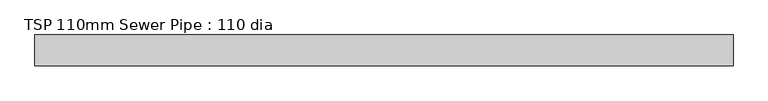
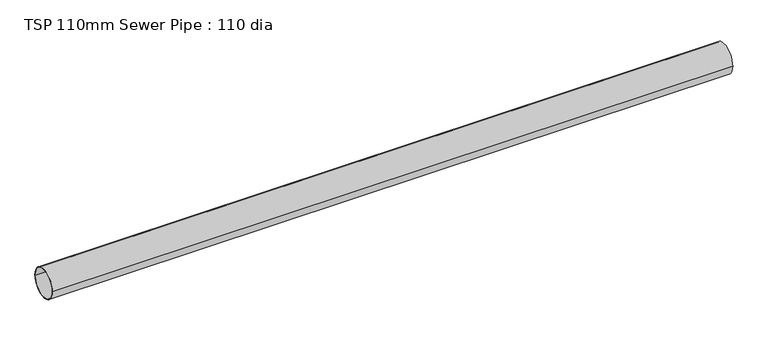
"""IFC4 building model written with IfcOpenShell, lengths in millimetres: flow terminal geometry, TSP 110mm Sewer Pipe : 110 dia."""

from ifc_helpers import new_model, si_unit, point, frame, origin, origin_2d, place, context, project, spatial, circle_curve, trimmed, segment, composite_curve, outline, extrude, source, transform, mapped, element, save


def tsp_110mm_sewer_pipe_110_dia_bab988ff(model_context):
    return source(origin(), model_context, "Body", "SweptSolid", [
        extrude(outline(composite_curve([segment(trimmed(circle_curve(origin_2d(), 55.0), [point((-55.0, 0.0))], [point((55.0, 0.0))], False, "CARTESIAN"), True, "CONTINUOUS"), segment(trimmed(circle_curve(origin_2d(), 55.0), [point((55.0, 0.0))], [point((-55.0, 0.0))], False, "CARTESIAN"), True, "CONTINUOUS")], self_intersect=False), holes=[composite_curve([segment(trimmed(circle_curve(origin_2d(), 52.0), [point((-52.0, 0.0))], [point((52.0, 0.0))], True, "CARTESIAN"), True, "CONTINUOUS"), segment(trimmed(circle_curve(origin_2d(), 52.0), [point((52.0, 0.0))], [point((-52.0, 0.0))], True, "CARTESIAN"), True, "CONTINUOUS")], self_intersect=False)]), frame((0.0, 0.0, 0.0), z_axis=(1.0, 0.0, 0.0), x_axis=(0.0, 1.0, 0.0)), (0.0, 0.0, 1.0), 2500.0),
    ])


if __name__ == "__main__":
    model = new_model("IFC4")
    model_context = context("Model", 3, world=origin())
    ifc_project = project(units=[si_unit("LENGTHUNIT", "METRE", prefix="MILLI")], contexts=[model_context])
    site = spatial("IfcSite", under=ifc_project)
    building = spatial("IfcBuilding", under=site)
    placement = place(None, origin())
    tsp_110mm_sewer_pipe_110_dia_shape = tsp_110mm_sewer_pipe_110_dia_bab988ff(model_context)
    element("IfcFlowTerminal", 1, ObjectType="TSP 110mm Sewer Pipe : 110 dia", at=placement, inside=building, context=model_context, shape_type="MappedRepresentation", body=[
        mapped(tsp_110mm_sewer_pipe_110_dia_shape, transform((0.0, 0.0, 0.0), x_axis=(1.0, 0.0, 0.0), y_axis=(0.0, 1.0, 0.0), z_axis=(0.0, 0.0, 1.0))),
    ])
    save(model, "model.ifc")

# Revit data of these elements
# Type "TSP 110mm Sewer Pipe : 110 dia"
#   Model = "TSP_110SWB"
#   Model = "TSP_110SWB"
#   Pipe length [instance default] = 1200 mm
#   Pipe dia = 110 mm
#   built-in parameter 1001306 [instance default] = 3.93701 (stored number, unit not read)
#   Default Elevation = 0
# Element 1 (IfcFlowTerminal, "TSP 110mm Sewer Pipe : 110 dia")
#   Pipe length = 2500 mm
#   built-in parameter 1001306 = 8.2021 (stored number, unit not read)
#   Materials on its faces: "Laminate, Brown, Matte"
# Materials
#   "Laminate, Brown, Matte": class "Plastic", colour RGB 128 64 0, transparency 0, Description = "Plastic Laminate - Red, Matte", Cost = 0
